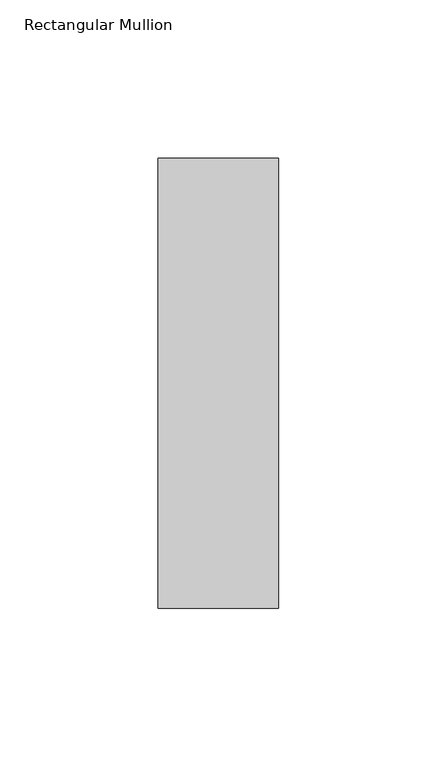
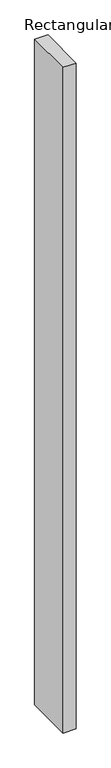
"""IFC4 building model written with IfcOpenShell, lengths in millimetres: member geometry, Rectangular Mullion : NLRS_21_CWM_hsb-regel 38x142_gen_rsf."""

from ifc_helpers import new_model, si_unit, frame, origin, place, context, project, spatial, polyline, outline, extrude, source, transform, mapped, element, save


def rectangular_mullion_b4280be7(model_context):
    return source(origin(), model_context, "Body", "SweptSolid", [
        extrude(outline(polyline([(-38.0, -71.0), (-38.0, 71.0), (0.0, 71.0), (0.0, -71.0), (-38.0, -71.0)])), frame((0.0, 0.0, -2038.0), z_axis=(0.0, 0.0, 1.0), x_axis=(1.0, 0.0, 0.0)), (0.0, 0.0, 1.0), 2038.0),
    ])


if __name__ == "__main__":
    model = new_model("IFC4")
    model_context = context("Model", 3, world=origin())
    ifc_project = project(units=[si_unit("LENGTHUNIT", "METRE", prefix="MILLI")], contexts=[model_context])
    site = spatial("IfcSite", under=ifc_project)
    building = spatial("IfcBuilding", under=site)
    placement = place(None, origin())
    rectangular_mullion_shape = rectangular_mullion_b4280be7(model_context)
    element("IfcMember", 1, ObjectType="Rectangular Mullion : NLRS_21_CWM_hsb-regel 38x142_gen_rsf", at=placement, inside=building, context=model_context, shape_type="MappedRepresentation", body=[
        mapped(rectangular_mullion_shape, transform((0.0, 0.0, 0.0), x_axis=(1.0, 0.0, 0.0), y_axis=(0.0, 1.0, 0.0), z_axis=(0.0, 0.0, 1.0))),
    ])
    save(model, "model.ifc")

# Revit data of these elements
# Type "Rectangular Mullion : NLRS_21_CWM_hsb-regel 38x142_gen_rsf"
#   Export Type to IFC As = "IfcWall"
#   Type IfcGUID = "07M7mRoiH1CR8m_RSKIwpF"
#   Assembly Code = "21.10"
#   built-in parameter 1007322 = 0.465879 (stored number, unit not read)
#   built-in parameter 1007321 = 0.062336 (stored number, unit not read)
#   built-in parameter 1007320 = 0.062336 (stored number, unit not read)
# Element 1 (IfcMember, "Rectangular Mullion : NLRS_21_CWM_hsb-regel 38x142_gen_rsf")
#   Materials on its faces: "NLRS_i2_hout naaldhout vuren_gen_rsf"
# Materials
#   "NLRS_i2_hout naaldhout vuren_gen_rsf": class "I - Hout", colour RGB 234 199 147, transparency 0, Keynote = "i2", Manufacturer = "Revit Standards Foundation", URL = "www.revitstandards.org", Description = "hout vuren", Cost = 0
